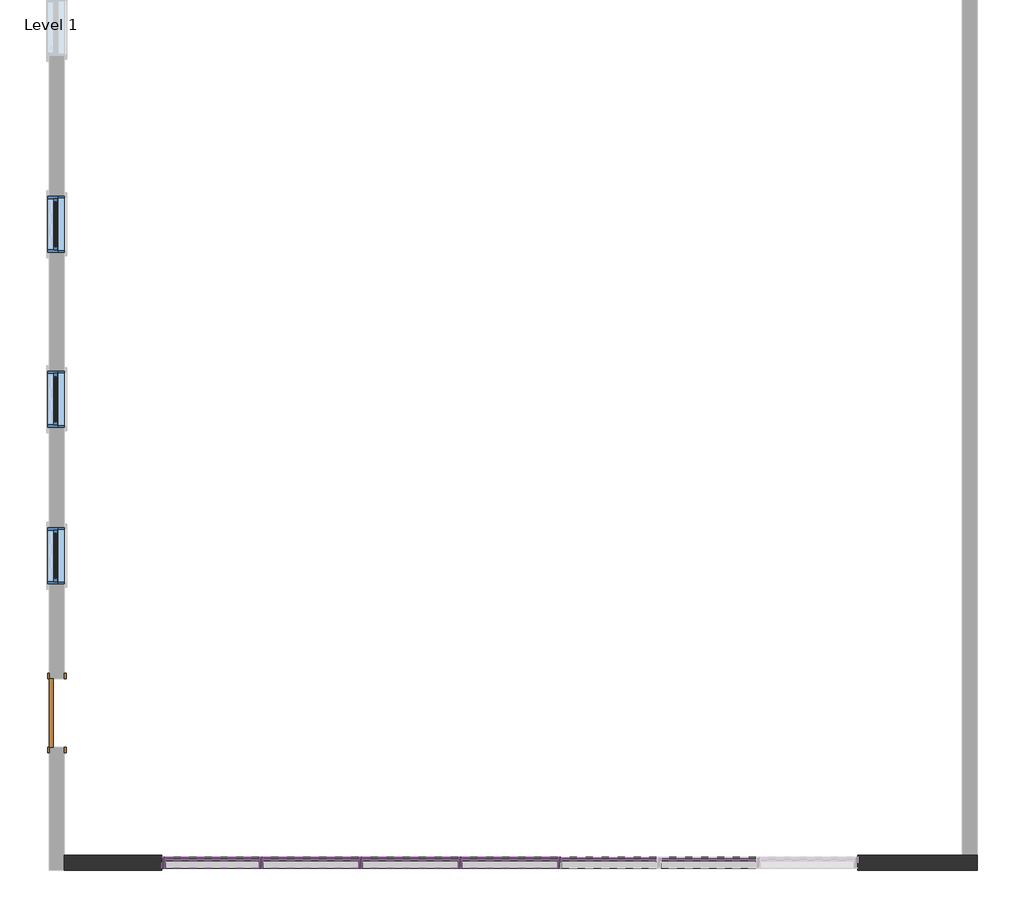
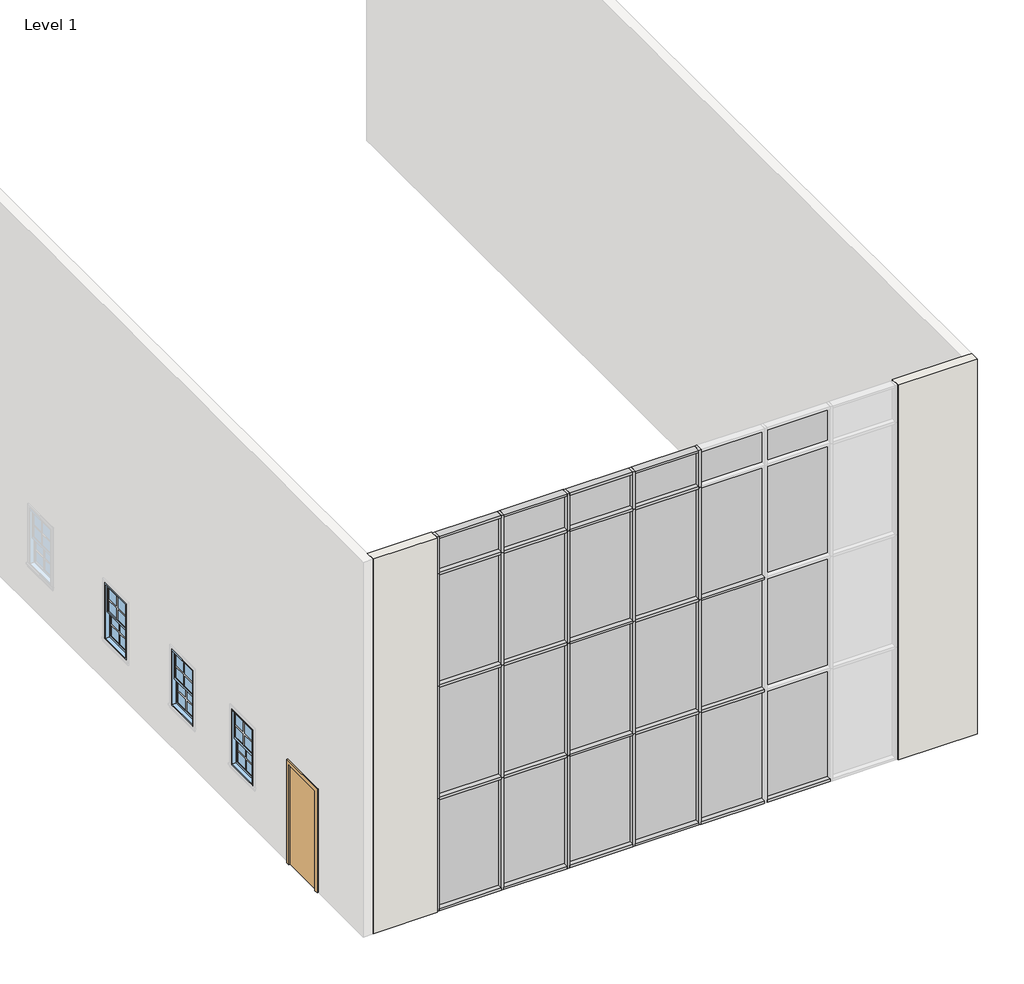
# One storey, part 1 of 2: 44 members, 24 plates, 3 windows, 1 door, 1 wall.
"""IFC4 building model written with IfcOpenShell, lengths in millimetres."""

import ifcopenshell
import ifcopenshell.guid

model = None  # the IFC model being written
_history = None  # IfcOwnerHistory: only IFC2X3 demands one
_inside = {}  # id of a spatial element -> (the spatial element, [elements in it])
_under = {}  # id of a project, library or spatial element -> (it, [spatial elements below it])
_declared = {}  # id of a project -> (the project, [libraries it declares])
_typed = {}  # id of a type object -> (the type object, [elements of that type])
_made_of = {}  # id of a material, layer set ... -> (it, [elements and type objects made of it])


def new_model(schema):
    """Start an empty IFC model of exactly this schema.

    Asked for "IFC4X3", IfcOpenShell would pick the latest addendum, in which some entities
    have other attributes; the version numbers below select the first issue.
    IFC2X3 requires an IfcOwnerHistory on every rooted entity: one is made here for all.
    """
    global model, _history
    if schema == "IFC4X3":
        model = ifcopenshell.file(schema_version=(4, 3, 0, 0))
    else:
        model = ifcopenshell.file(schema=schema)
    _inside.clear()
    _under.clear()
    _declared.clear()
    _typed.clear()
    _made_of.clear()
    _history = None
    if model.schema == "IFC2X3":
        org = make("IfcOrganization", Name="unknown")
        user = make(
            "IfcPersonAndOrganization",
            ThePerson=make("IfcPerson", FamilyName="unknown"),
            TheOrganization=org,
        )
        app = make(
            "IfcApplication",
            ApplicationDeveloper=org,
            Version="unknown",
            ApplicationFullName="unknown",
            ApplicationIdentifier="unknown",
        )
        _history = make(
            "IfcOwnerHistory",
            OwningUser=user,
            OwningApplication=app,
            ChangeAction="ADDED",
            CreationDate=0,
        )
    return model


def make(cls, **values):
    """One entity of the class cls with the attributes given. An attribute that is None is left unset."""
    return model.create_entity(
        cls, **{name: value for name, value in values.items() if value is not None}
    )


def rooted(cls, **values):
    """An entity with a GlobalId (a new one), such as an element, a storey or a relation."""
    return make(cls, GlobalId=ifcopenshell.guid.new(), OwnerHistory=_history, **values)


def si_unit(unit_type, name, prefix=None):
    """IfcSIUnit, for example si_unit("LENGTHUNIT", "METRE", prefix="MILLI")."""
    return make("IfcSIUnit", UnitType=unit_type, Prefix=prefix, Name=name)


def assignment(units):
    """IfcUnitAssignment: the units of a project."""
    return None if units is None else make("IfcUnitAssignment", Units=units)


def point(xyz):
    """IfcCartesianPoint."""
    return None if xyz is None else make("IfcCartesianPoint", Coordinates=xyz)


def direction(xyz):
    """IfcDirection."""
    return None if xyz is None else make("IfcDirection", DirectionRatios=xyz)


def frame(location, z_axis=None, x_axis=None):
    """IfcAxis2Placement3D, a coordinate frame: its origin and axes. An axis left out is left unset."""
    return make(
        "IfcAxis2Placement3D",
        Location=point(location),
        Axis=direction(z_axis),
        RefDirection=direction(x_axis),
    )


def origin():
    """The frame at (0, 0, 0) with its axes left unset."""
    return frame((0.0, 0.0, 0.0))


def origin_with_axes():
    """The frame at (0, 0, 0) with the z axis (0, 0, 1) and the x axis (1, 0, 0) written out."""
    return frame((0.0, 0.0, 0.0), z_axis=(0.0, 0.0, 1.0), x_axis=(1.0, 0.0, 0.0))


def place(relative_to, where):
    """IfcLocalPlacement: puts the frame where relative to a parent placement (None: the world)."""
    return make(
        "IfcLocalPlacement", PlacementRelTo=relative_to, RelativePlacement=where
    )


def context(
    kind, dimensions, precision=None, world=None, true_north=None, identifier=None
):
    """IfcGeometricRepresentationContext, for example the 3D "Model" context."""
    return make(
        "IfcGeometricRepresentationContext",
        ContextIdentifier=identifier,
        ContextType=kind,
        CoordinateSpaceDimension=dimensions,
        Precision=precision,
        WorldCoordinateSystem=world,
        TrueNorth=true_north,
    )


def project(units=None, contexts=None):
    """IfcProject with its units and contexts."""
    return rooted(
        "IfcProject",
        Name="project",
        RepresentationContexts=contexts,
        UnitsInContext=assignment(units),
    )


def spatial(cls, under=None, at=None, **own):
    """A site, building, storey or space (cls), placed at a placement, below another one or the project."""
    s = rooted(cls, ObjectPlacement=at, **own)
    if under is not None:
        _under.setdefault(under.id(), (under, []))[1].append(s)
    return s


def polyline(points):
    """IfcPolyline through the points."""
    return make("IfcPolyline", Points=[point(p) for p in points])


def outline(outer, holes=None, kind="AREA"):
    """IfcArbitraryClosedProfileDef: a profile drawn as a closed curve; with holes, ...WithVoids."""
    if holes is None:
        return make("IfcArbitraryClosedProfileDef", ProfileType=kind, OuterCurve=outer)
    return make(
        "IfcArbitraryProfileDefWithVoids",
        ProfileType=kind,
        OuterCurve=outer,
        InnerCurves=holes,
    )


def extrude(swept, where, along, depth):
    """IfcExtrudedAreaSolid: the profile swept, set in the frame where, extruded along a direction by depth."""
    return make(
        "IfcExtrudedAreaSolid",
        SweptArea=swept,
        Position=where,
        ExtrudedDirection=direction(along),
        Depth=depth,
    )


def faces_of(points, faces, orient=None, outer=None):
    """IfcFace entities. A face is a list of loops; a loop is a list of indices into points, from 0.

    orient and outer hold one flag for each loop. By default every Orientation is true, the
    first loop of a face is its IfcFaceOuterBound and the others are IfcFaceBound.
    """
    made = []
    for i, loops in enumerate(faces):
        bounds = []
        for j, loop in enumerate(loops):
            is_outer = j == 0 if outer is None else outer[i][j]
            bounds.append(
                make(
                    "IfcFaceOuterBound" if is_outer else "IfcFaceBound",
                    Bound=make("IfcPolyLoop", Polygon=[points[k] for k in loop]),
                    Orientation=True if orient is None else orient[i][j],
                )
            )
        made.append(make("IfcFace", Bounds=bounds))
    return made


def faceted_brep(points, faces, orient=None, outer=None, voids=None):
    """IfcFacetedBrep: a solid bounded by flat faces; with voids (closed shells), ...WithVoids."""
    shared = [point(p) for p in points]
    hull = make("IfcClosedShell", CfsFaces=faces_of(shared, faces, orient, outer))
    if voids is None:
        return make("IfcFacetedBrep", Outer=hull)
    return make(
        "IfcFacetedBrepWithVoids",
        Outer=hull,
        Voids=[
            make(cls, CfsFaces=faces_of(shared, fs, o, b)) for cls, fs, o, b in voids
        ],
    )


def shape(context_of_items, identifier, shape_type, items):
    """IfcShapeRepresentation: the items that make up one representation, for example the "Body"."""
    return make(
        "IfcShapeRepresentation",
        ContextOfItems=context_of_items,
        RepresentationIdentifier=identifier,
        RepresentationType=shape_type,
        Items=items,
    )


def source(mapping_origin, context_of_items, identifier, shape_type, items):
    """IfcRepresentationMap: a shape defined once, which mapped items show again and again."""
    return make(
        "IfcRepresentationMap",
        MappingOrigin=mapping_origin,
        MappedRepresentation=shape(context_of_items, identifier, shape_type, items),
    )


def transform(
    local_origin,
    x_axis=None,
    y_axis=None,
    z_axis=None,
    scale=None,
    scale2=None,
    scale3=None,
    uniform=True,
):
    """IfcCartesianTransformationOperator3D, or its non-uniform kind. x_axis, y_axis, z_axis: its Axis1, 2, 3."""
    if uniform:
        return make(
            "IfcCartesianTransformationOperator3D",
            Axis1=direction(x_axis),
            Axis2=direction(y_axis),
            LocalOrigin=point(local_origin),
            Scale=scale,
            Axis3=direction(z_axis),
        )
    return make(
        "IfcCartesianTransformationOperator3DnonUniform",
        Axis1=direction(x_axis),
        Axis2=direction(y_axis),
        LocalOrigin=point(local_origin),
        Scale=scale,
        Axis3=direction(z_axis),
        Scale2=scale2,
        Scale3=scale3,
    )


def mapped(mapping_source, mapping_target):
    """IfcMappedItem: shows the shape of a source again, moved by a transform."""
    return make(
        "IfcMappedItem", MappingSource=mapping_source, MappingTarget=mapping_target
    )


def made_of(thing, what):
    """Note that an element or type object is made of a material, layer set ...; save() writes the relation."""
    if what is not None:
        _made_of.setdefault(what.id(), (what, []))[1].append(thing)
    return thing


def element(
    cls,
    number,
    at=None,
    inside=None,
    cuts=None,
    type_object=None,
    material=None,
    context=None,
    identifier="Body",
    shape_type=None,
    held_by="IfcProductDefinitionShape",
    body=None,
    shapes=None,
    **own,
):
    """One element of the class cls, such as IfcWall. Its Tag is "e" and its number.

    at: its placement. inside: the storey or other place that contains it. cuts: it is an
    opening in that element (IfcRelVoidsElement). A single representation is given by context,
    identifier, shape_type and body (its items); several are given by shapes. held_by: the class
    of the entity that holds the representations. save() writes the other relations.
    """
    e = rooted(cls, Tag="e%d" % number, ObjectPlacement=at, **own)
    if body is not None:
        shapes = [shape(context, identifier, shape_type, body)]
    if shapes is not None:
        e.Representation = make(held_by, Representations=shapes)
    if inside is not None:
        _inside.setdefault(inside.id(), (inside, []))[1].append(e)
    if cuts is not None:
        rooted(
            "IfcRelVoidsElement", RelatingBuildingElement=cuts, RelatedOpeningElement=e
        )
    if type_object is not None:
        _typed.setdefault(type_object.id(), (type_object, []))[1].append(e)
    return made_of(e, material)


def aggregate(whole, parts):
    """IfcRelAggregates: a whole, such as a stair, and the parts it consists of."""
    return rooted("IfcRelAggregates", RelatingObject=whole, RelatedObjects=parts)


def save(model, path):
    """Write the relations noted so far, then the file.

    IfcRelAggregates (storeys below a building ...), IfcRelContainedInSpatialStructure (elements
    in a storey), IfcRelDefinesByType, IfcRelAssociatesMaterial and IfcRelDeclares: one each for
    every whole, place, type object, material and project.
    """
    for whole, parts in _under.values():
        aggregate(whole, parts)
    for where, things in _inside.values():
        rooted(
            "IfcRelContainedInSpatialStructure",
            RelatedElements=things,
            RelatingStructure=where,
        )
    for kind, things in _typed.values():
        rooted("IfcRelDefinesByType", RelatedObjects=things, RelatingType=kind)
    for what, things in _made_of.values():
        rooted("IfcRelAssociatesMaterial", RelatedObjects=things, RelatingMaterial=what)
    for by, libraries in _declared.values():
        rooted("IfcRelDeclares", RelatingContext=by, RelatedDefinitions=libraries)
    model.write(path)


def m_single_flush_0915_x_2134mm_6a9e8738(model_context):
    return source(origin(), model_context, "Body", "SweptSolid", [
        extrude(outline(polyline([(2210.0, -533.5), (0.0, -533.5), (0.0, -457.5), (2134.0, -457.5), (2134.0, 457.5), (0.0, 457.5), (0.0, 533.5), (2210.0, 533.5), (2210.0, -533.5)])), frame((0.0, 100.0, 0.0), z_axis=(0.0, 1.0, 0.0), x_axis=(0.0, 0.0, 1.0)), (0.0, 0.0, 1.0), 25.0),
        extrude(outline(polyline([(2210.0, 533.5), (2210.0, -533.5), (0.0, -533.5), (0.0, -457.5), (2134.0, -457.5), (2134.0, 457.5), (0.0, 457.5), (0.0, 533.5), (2210.0, 533.5)])), frame((0.0, -125.0, 0.0), z_axis=(0.0, 1.0, 0.0), x_axis=(0.0, 0.0, 1.0)), (0.0, 0.0, 1.0), 25.0),
        extrude(outline(polyline([(457.5, 49.0), (-457.5, 49.0), (-457.5, 100.0), (457.5, 100.0), (457.5, 49.0)])), origin_with_axes(), (0.0, 0.0, 1.0), 2134.0),
    ])


def rectangular_mullion_50mm_x_150mm_302a0cfa(model_context):
    return source(origin(), model_context, "Body", "SweptSolid", [
        extrude(outline(polyline([(0.0, 75.0), (0.0, -75.0), (-50.0, -75.0), (-50.0, 75.0), (0.0, 75.0)])), frame((0.0, 0.0, -1253.5714288), z_axis=(0.0, 0.0, 1.0), x_axis=(1.0, 0.0, 0.0)), (0.0, 0.0, 1.0), 1253.5714288),
    ])


def rectangular_mullion_50mm_x_150mm_11a5ee59(model_context):
    return source(origin(), model_context, "Body", "SweptSolid", [
        extrude(outline(polyline([(0.0, 75.0), (0.0, -75.0), (-50.0, -75.0), (-50.0, 75.0), (0.0, 75.0)])), frame((0.0, 0.0, -1278.5714285), z_axis=(0.0, 0.0, 1.0), x_axis=(1.0, 0.0, 0.0)), (0.0, 0.0, 1.0), 1278.5714285),
    ])


def rectangular_mullion_50mm_x_150mm_46426fc7(model_context):
    return source(origin(), model_context, "Body", "SweptSolid", [
        extrude(outline(polyline([(25.0, 75.0), (25.0, -75.0), (-25.0, -75.0), (-25.0, 75.0), (25.0, 75.0)])), frame((0.0, 0.0, -1253.5714288), z_axis=(0.0, 0.0, 1.0), x_axis=(1.0, 0.0, 0.0)), (0.0, 0.0, 1.0), 1253.5714288),
    ])


def rectangular_mullion_50mm_x_150mm_f38f42f6(model_context):
    return source(origin(), model_context, "Body", "SweptSolid", [
        extrude(outline(polyline([(25.0, 75.0), (25.0, -75.0), (-25.0, -75.0), (-25.0, 75.0), (25.0, 75.0)])), frame((0.0, 0.0, -1278.5714285), z_axis=(0.0, 0.0, 1.0), x_axis=(1.0, 0.0, 0.0)), (0.0, 0.0, 1.0), 1278.5714285),
    ])


def rectangular_mullion_50mm_x_150mm_6225e4e3(model_context):
    return source(origin(), model_context, "Body", "SweptSolid", [
        extrude(outline(polyline([(25.0, 75.0), (25.0, -75.0), (-25.0, -75.0), (-25.0, 75.0), (25.0, 75.0)])), frame((0.0, 0.0, -2400.0), z_axis=(0.0, 0.0, 1.0), x_axis=(1.0, 0.0, 0.0)), (0.0, 0.0, 1.0), 2400.0),
    ])


def rectangular_mullion_50mm_x_150mm_662c37b1(model_context):
    return source(origin(), model_context, "Body", "SweptSolid", [
        extrude(outline(polyline([(0.0, 75.0), (0.0, -75.0), (-50.0, -75.0), (-50.0, 75.0), (0.0, 75.0)])), frame((0.0, 0.0, -2400.0), z_axis=(0.0, 0.0, 1.0), x_axis=(1.0, 0.0, 0.0)), (0.0, 0.0, 1.0), 2400.0),
    ])


def rectangular_mullion_50mm_x_150mm_14f10ac7(model_context):
    return source(origin(), model_context, "Body", "SweptSolid", [
        extrude(outline(polyline([(25.0, 75.0), (25.0, -75.0), (-25.0, -75.0), (-25.0, 75.0), (25.0, 75.0)])), frame((0.0, 0.0, -800.0), z_axis=(0.0, 0.0, 1.0), x_axis=(1.0, 0.0, 0.0)), (0.0, 0.0, 1.0), 800.0),
    ])


def rectangular_mullion_50mm_x_150mm_6ffebc0f(model_context):
    return source(origin(), model_context, "Body", "SweptSolid", [
        extrude(outline(polyline([(0.0, 75.0), (0.0, -75.0), (-50.0, -75.0), (-50.0, 75.0), (0.0, 75.0)])), frame((0.0, 0.0, -800.0), z_axis=(0.0, 0.0, 1.0), x_axis=(1.0, 0.0, 0.0)), (0.0, 0.0, 1.0), 800.0),
    ])


def system_panel_glazed_b60b372a(model_context):
    return source(origin(), model_context, "Body", "SweptSolid", [
        extrude(outline(polyline([(626.7857144, 24.5), (-626.7857144, 24.5), (-626.7857144, 49.5), (626.7857144, 49.5), (626.7857144, 24.5)])), origin_with_axes(), (0.0, 0.0, 1.0), 2325.0),
    ])


def system_panel_glazed_fd68b2ce(model_context):
    return source(origin(), model_context, "Body", "SweptSolid", [
        extrude(outline(polyline([(639.2857142, 24.5), (-639.2857142, 24.5), (-639.2857142, 49.5), (639.2857142, 49.5), (639.2857142, 24.5)])), origin_with_axes(), (0.0, 0.0, 1.0), 2325.0),
    ])


def system_panel_glazed_eec4e8b3(model_context):
    return source(origin(), model_context, "Body", "SweptSolid", [
        extrude(outline(polyline([(626.7857144, 24.5), (-626.7857144, 24.5), (-626.7857144, 49.5), (626.7857144, 49.5), (626.7857144, 24.5)])), origin_with_axes(), (0.0, 0.0, 1.0), 2350.0),
    ])


def system_panel_glazed_5b896d3e(model_context):
    return source(origin(), model_context, "Body", "SweptSolid", [
        extrude(outline(polyline([(639.2857142, 24.5), (-639.2857142, 24.5), (-639.2857142, 49.5), (639.2857142, 49.5), (639.2857142, 24.5)])), origin_with_axes(), (0.0, 0.0, 1.0), 2350.0),
    ])


def system_panel_glazed_efd17426(model_context):
    return source(origin(), model_context, "Body", "SweptSolid", [
        extrude(outline(polyline([(626.7857144, 24.5), (-626.7857144, 24.5), (-626.7857144, 49.5), (626.7857144, 49.5), (626.7857144, 24.5)])), origin_with_axes(), (0.0, 0.0, 1.0), 725.0),
    ])


def system_panel_glazed_74448b90(model_context):
    return source(origin(), model_context, "Body", "SweptSolid", [
        extrude(outline(polyline([(639.2857142, 24.5), (-639.2857142, 24.5), (-639.2857142, 49.5), (639.2857142, 49.5), (639.2857142, 24.5)])), origin_with_axes(), (0.0, 0.0, 1.0), 725.0),
    ])


def m_window_double_hung_750_x_1200mm_41070976(model_context):
    return source(origin(), model_context, "Body", "SweptSolid", [
        extrude(outline(polyline([(298.8, 30.15), (298.8, 23.8), (-298.8, 23.8), (-298.8, 30.15), (298.8, 30.15)])), frame((0.0, 0.0, 990.6), z_axis=(0.0, 0.0, 1.0), x_axis=(1.0, 0.0, 0.0)), (0.0, 0.0, 1.0), 501.575),
        extrude(outline(polyline([(-298.8, 17.45), (298.8, 17.45), (298.8, 11.1), (-298.8, 11.1), (-298.8, 17.45)])), frame((0.0, 0.0, 990.6), z_axis=(0.0, 0.0, 1.0), x_axis=(1.0, 0.0, 0.0)), (0.0, 0.0, 1.0), 501.575),
        extrude(outline(polyline([(298.8, 74.6), (298.8, 68.25), (-298.8, 68.25), (-298.8, 74.6), (298.8, 74.6)])), frame((0.0, 0.0, 1536.625), z_axis=(0.0, 0.0, 1.0), x_axis=(1.0, 0.0, 0.0)), (0.0, 0.0, 1.0), 501.575),
        extrude(outline(polyline([(-298.8, 61.9), (298.8, 61.9), (298.8, 55.55), (-298.8, 55.55), (-298.8, 61.9)])), frame((0.0, 0.0, 1536.625), z_axis=(0.0, 0.0, 1.0), x_axis=(1.0, 0.0, 0.0)), (0.0, 0.0, 1.0), 501.575),
        extrude(outline(polyline([(1536.625, -343.25), (946.15, -343.25), (946.15, 343.25), (1536.625, 343.25), (1536.625, -343.25)]), holes=[polyline([(1492.175, 298.8), (990.6, 298.8), (990.6, -298.8), (1492.175, -298.8), (1492.175, 298.8)])]), frame((0.0, -1.6, 0.0), z_axis=(0.0, 1.0, 0.0), x_axis=(0.0, 0.0, 1.0)), (0.0, 0.0, 1.0), 44.45),
        extrude(outline(polyline([(2082.65, -343.25), (1492.175, -343.25), (1492.175, 343.25), (2082.65, 343.25), (2082.65, -343.25)]), holes=[polyline([(2038.2, 298.8), (1536.625, 298.8), (1536.625, -298.8), (2038.2, -298.8), (2038.2, 298.8)])]), frame((0.0, 42.85, 0.0), z_axis=(0.0, 1.0, 0.0), x_axis=(0.0, 0.0, 1.0)), (0.0, 0.0, 1.0), 44.45),
        extrude(outline(polyline([(2114.4, -375.0), (914.4, -375.0), (914.4, 375.0), (2114.4, 375.0), (2114.4, -375.0)]), holes=[polyline([(2082.65, 343.25), (946.15, 343.25), (946.15, -343.25), (2082.65, -343.25), (2082.65, 343.25)])]), frame((0.0, -14.3, 0.0), z_axis=(0.0, 1.0, 0.0), x_axis=(0.0, 0.0, 1.0)), (0.0, 0.0, 1.0), 133.35),
        extrude(outline(polyline([(2114.4, 375.0), (2114.4, -375.0), (914.4, -375.0), (914.4, 375.0), (2114.4, 375.0)]), holes=[polyline([(2095.35, 355.95), (933.45, 355.95), (933.45, -355.95), (2095.35, -355.95), (2095.35, 355.95)])]), frame((0.0, -100.0, 0.0), z_axis=(0.0, 1.0, 0.0), x_axis=(0.0, 0.0, 1.0)), (0.0, 0.0, 1.0), 85.7),
    ])


model = new_model("IFC4")

# Units and contexts
model_context = context("Model", 3, world=origin())
ifc_project = project(units=[si_unit("LENGTHUNIT", "METRE", prefix="MILLI")], contexts=[model_context])

# Site, building, storey
site = spatial("IfcSite", under=ifc_project)
building = spatial("IfcBuilding", under=site)
storey = spatial("IfcBuildingStorey", under=building, Name="Level 1", Elevation=0.0)

# Door
placement = place(None, origin())
m_single_flush_0915_x_2134mm_shape = m_single_flush_0915_x_2134mm_6a9e8738(model_context)
element("IfcDoor", 1, ObjectType="M_Single-Flush : 0915 x 2134mm", at=placement, inside=storey, context=model_context, shape_type="MappedRepresentation", body=[
    mapped(m_single_flush_0915_x_2134mm_shape, transform((-6967.834392, -6666.9793434, 0.0), x_axis=(0.0, 1.0, 0.0), y_axis=(-1.0, 0.0, 0.0), z_axis=(0.0, 0.0, 1.0))),
])

# Members
rectangular_mullion_50mm_x_150mm_shape = rectangular_mullion_50mm_x_150mm_302a0cfa(model_context)
element("IfcMember", 2, ObjectType="Rectangular Mullion : 50mm x 150mm", at=placement, inside=storey, context=model_context, shape_type="MappedRepresentation", body=[
    mapped(rectangular_mullion_50mm_x_150mm_shape, transform((-5517.834392, -8666.9793434, 0.0), x_axis=(0.0, 0.0, -1.0), y_axis=(0.0, -1.0, 0.0), z_axis=(-1.0, 0.0, 0.0))),
])
rectangular_mullion_50mm_x_150mm_2_shape = rectangular_mullion_50mm_x_150mm_11a5ee59(model_context)
element("IfcMember", 3, ObjectType="Rectangular Mullion : 50mm x 150mm", at=placement, inside=storey, context=model_context, shape_type="MappedRepresentation", body=[
    mapped(rectangular_mullion_50mm_x_150mm_2_shape, transform((-4214.2629632, -8666.9793434, 0.0), x_axis=(0.0, 0.0, -1.0), y_axis=(0.0, -1.0, 0.0), z_axis=(-1.0, 0.0, 0.0))),
])
element("IfcMember", 4, ObjectType="Rectangular Mullion : 50mm x 150mm", at=placement, inside=storey, context=model_context, shape_type="MappedRepresentation", body=[
    mapped(rectangular_mullion_50mm_x_150mm_2_shape, transform((-2885.6915347, -8666.9793434, 0.0), x_axis=(0.0, 0.0, -1.0), y_axis=(0.0, -1.0, 0.0), z_axis=(-1.0, 0.0, 0.0))),
])
element("IfcMember", 5, ObjectType="Rectangular Mullion : 50mm x 150mm", at=placement, inside=storey, context=model_context, shape_type="MappedRepresentation", body=[
    mapped(rectangular_mullion_50mm_x_150mm_2_shape, transform((-1557.1201062, -8666.9793434, 0.0), x_axis=(0.0, 0.0, -1.0), y_axis=(0.0, -1.0, 0.0), z_axis=(-1.0, 0.0, 0.0))),
])
element("IfcMember", 6, ObjectType="Rectangular Mullion : 50mm x 150mm", at=placement, inside=storey, context=model_context, shape_type="MappedRepresentation", body=[
    mapped(rectangular_mullion_50mm_x_150mm_2_shape, transform((-228.5486777, -8666.9793434, 0.0), x_axis=(0.0, 0.0, -1.0), y_axis=(0.0, -1.0, 0.0), z_axis=(-1.0, 0.0, 0.0))),
])
element("IfcMember", 7, ObjectType="Rectangular Mullion : 50mm x 150mm", at=placement, inside=storey, context=model_context, shape_type="MappedRepresentation", body=[
    mapped(rectangular_mullion_50mm_x_150mm_2_shape, transform((1100.0227508, -8666.9793434, 0.0), x_axis=(0.0, 0.0, -1.0), y_axis=(0.0, -1.0, 0.0), z_axis=(-1.0, 0.0, 0.0))),
])
rectangular_mullion_50mm_x_150mm_3_shape = rectangular_mullion_50mm_x_150mm_46426fc7(model_context)
element("IfcMember", 8, ObjectType="Rectangular Mullion : 50mm x 150mm", at=placement, inside=storey, context=model_context, shape_type="MappedRepresentation", body=[
    mapped(rectangular_mullion_50mm_x_150mm_3_shape, transform((-4264.2629632, -8666.9793434, 2400.0), x_axis=(0.0, 0.0, 1.0), y_axis=(0.0, -1.0, 0.0), z_axis=(1.0, 0.0, 0.0))),
])
element("IfcMember", 9, ObjectType="Rectangular Mullion : 50mm x 150mm", at=placement, inside=storey, context=model_context, shape_type="MappedRepresentation", body=[
    mapped(rectangular_mullion_50mm_x_150mm_3_shape, transform((-4264.2629632, -8666.9793434, 4800.0), x_axis=(0.0, 0.0, 1.0), y_axis=(0.0, -1.0, 0.0), z_axis=(1.0, 0.0, 0.0))),
])
element("IfcMember", 10, ObjectType="Rectangular Mullion : 50mm x 150mm", at=placement, inside=storey, context=model_context, shape_type="MappedRepresentation", body=[
    mapped(rectangular_mullion_50mm_x_150mm_3_shape, transform((-4264.2629632, -8666.9793434, 7200.0), x_axis=(0.0, 0.0, 1.0), y_axis=(0.0, -1.0, 0.0), z_axis=(1.0, 0.0, 0.0))),
])
rectangular_mullion_50mm_x_150mm_4_shape = rectangular_mullion_50mm_x_150mm_f38f42f6(model_context)
element("IfcMember", 11, ObjectType="Rectangular Mullion : 50mm x 150mm", at=placement, inside=storey, context=model_context, shape_type="MappedRepresentation", body=[
    mapped(rectangular_mullion_50mm_x_150mm_4_shape, transform((-2935.6915347, -8666.9793434, 2400.0), x_axis=(0.0, 0.0, 1.0), y_axis=(0.0, -1.0, 0.0), z_axis=(1.0, 0.0, 0.0))),
])
element("IfcMember", 12, ObjectType="Rectangular Mullion : 50mm x 150mm", at=placement, inside=storey, context=model_context, shape_type="MappedRepresentation", body=[
    mapped(rectangular_mullion_50mm_x_150mm_4_shape, transform((-1607.1201062, -8666.9793434, 2400.0), x_axis=(0.0, 0.0, 1.0), y_axis=(0.0, -1.0, 0.0), z_axis=(1.0, 0.0, 0.0))),
])
element("IfcMember", 13, ObjectType="Rectangular Mullion : 50mm x 150mm", at=placement, inside=storey, context=model_context, shape_type="MappedRepresentation", body=[
    mapped(rectangular_mullion_50mm_x_150mm_4_shape, transform((-278.5486777, -8666.9793434, 2400.0), x_axis=(0.0, 0.0, 1.0), y_axis=(0.0, -1.0, 0.0), z_axis=(1.0, 0.0, 0.0))),
])
element("IfcMember", 14, ObjectType="Rectangular Mullion : 50mm x 150mm", at=placement, inside=storey, context=model_context, shape_type="MappedRepresentation", body=[
    mapped(rectangular_mullion_50mm_x_150mm_4_shape, transform((1050.0227508, -8666.9793434, 2400.0), x_axis=(0.0, 0.0, 1.0), y_axis=(0.0, -1.0, 0.0), z_axis=(1.0, 0.0, 0.0))),
])
element("IfcMember", 15, ObjectType="Rectangular Mullion : 50mm x 150mm", at=placement, inside=storey, context=model_context, shape_type="MappedRepresentation", body=[
    mapped(rectangular_mullion_50mm_x_150mm_4_shape, transform((-2935.6915347, -8666.9793434, 4800.0), x_axis=(0.0, 0.0, 1.0), y_axis=(0.0, -1.0, 0.0), z_axis=(1.0, 0.0, 0.0))),
])
element("IfcMember", 16, ObjectType="Rectangular Mullion : 50mm x 150mm", at=placement, inside=storey, context=model_context, shape_type="MappedRepresentation", body=[
    mapped(rectangular_mullion_50mm_x_150mm_4_shape, transform((-1607.1201062, -8666.9793434, 4800.0), x_axis=(0.0, 0.0, 1.0), y_axis=(0.0, -1.0, 0.0), z_axis=(1.0, 0.0, 0.0))),
])
element("IfcMember", 17, ObjectType="Rectangular Mullion : 50mm x 150mm", at=placement, inside=storey, context=model_context, shape_type="MappedRepresentation", body=[
    mapped(rectangular_mullion_50mm_x_150mm_4_shape, transform((-278.5486777, -8666.9793434, 4800.0), x_axis=(0.0, 0.0, 1.0), y_axis=(0.0, -1.0, 0.0), z_axis=(1.0, 0.0, 0.0))),
])
element("IfcMember", 18, ObjectType="Rectangular Mullion : 50mm x 150mm", at=placement, inside=storey, context=model_context, shape_type="MappedRepresentation", body=[
    mapped(rectangular_mullion_50mm_x_150mm_4_shape, transform((1050.0227508, -8666.9793434, 4800.0), x_axis=(0.0, 0.0, 1.0), y_axis=(0.0, -1.0, 0.0), z_axis=(1.0, 0.0, 0.0))),
])
element("IfcMember", 19, ObjectType="Rectangular Mullion : 50mm x 150mm", at=placement, inside=storey, context=model_context, shape_type="MappedRepresentation", body=[
    mapped(rectangular_mullion_50mm_x_150mm_4_shape, transform((-1607.1201062, -8666.9793434, 7200.0), x_axis=(0.0, 0.0, 1.0), y_axis=(0.0, -1.0, 0.0), z_axis=(1.0, 0.0, 0.0))),
])
element("IfcMember", 20, ObjectType="Rectangular Mullion : 50mm x 150mm", at=placement, inside=storey, context=model_context, shape_type="MappedRepresentation", body=[
    mapped(rectangular_mullion_50mm_x_150mm_4_shape, transform((-278.5486777, -8666.9793434, 7200.0), x_axis=(0.0, 0.0, 1.0), y_axis=(0.0, -1.0, 0.0), z_axis=(1.0, 0.0, 0.0))),
])
element("IfcMember", 21, ObjectType="Rectangular Mullion : 50mm x 150mm", at=placement, inside=storey, context=model_context, shape_type="MappedRepresentation", body=[
    mapped(rectangular_mullion_50mm_x_150mm_4_shape, transform((-2935.6915347, -8666.9793434, 7200.0), x_axis=(0.0, 0.0, 1.0), y_axis=(0.0, -1.0, 0.0), z_axis=(1.0, 0.0, 0.0))),
])
rectangular_mullion_50mm_x_150mm_5_shape = rectangular_mullion_50mm_x_150mm_6225e4e3(model_context)
element("IfcMember", 22, ObjectType="Rectangular Mullion : 50mm x 150mm", at=placement, inside=storey, context=model_context, shape_type="MappedRepresentation", body=[
    mapped(rectangular_mullion_50mm_x_150mm_5_shape, transform((-4239.2629632, -8666.9793434, 0.0), x_axis=(1.0, 0.0, 0.0), y_axis=(0.0, -1.0, 0.0), z_axis=(0.0, 0.0, -1.0))),
])
element("IfcMember", 23, ObjectType="Rectangular Mullion : 50mm x 150mm", at=placement, inside=storey, context=model_context, shape_type="MappedRepresentation", body=[
    mapped(rectangular_mullion_50mm_x_150mm_5_shape, transform((-2910.6915347, -8666.9793434, 0.0), x_axis=(1.0, 0.0, 0.0), y_axis=(0.0, -1.0, 0.0), z_axis=(0.0, 0.0, -1.0))),
])
element("IfcMember", 24, ObjectType="Rectangular Mullion : 50mm x 150mm", at=placement, inside=storey, context=model_context, shape_type="MappedRepresentation", body=[
    mapped(rectangular_mullion_50mm_x_150mm_5_shape, transform((-1582.1201062, -8666.9793434, 0.0), x_axis=(1.0, 0.0, 0.0), y_axis=(0.0, -1.0, 0.0), z_axis=(0.0, 0.0, -1.0))),
])
element("IfcMember", 25, ObjectType="Rectangular Mullion : 50mm x 150mm", at=placement, inside=storey, context=model_context, shape_type="MappedRepresentation", body=[
    mapped(rectangular_mullion_50mm_x_150mm_5_shape, transform((-253.5486777, -8666.9793434, 0.0), x_axis=(1.0, 0.0, 0.0), y_axis=(0.0, -1.0, 0.0), z_axis=(0.0, 0.0, -1.0))),
])
element("IfcMember", 26, ObjectType="Rectangular Mullion : 50mm x 150mm", at=placement, inside=storey, context=model_context, shape_type="MappedRepresentation", body=[
    mapped(rectangular_mullion_50mm_x_150mm_5_shape, transform((-4239.2629632, -8666.9793434, 2400.0), x_axis=(1.0, 0.0, 0.0), y_axis=(0.0, -1.0, 0.0), z_axis=(0.0, 0.0, -1.0))),
])
element("IfcMember", 27, ObjectType="Rectangular Mullion : 50mm x 150mm", at=placement, inside=storey, context=model_context, shape_type="MappedRepresentation", body=[
    mapped(rectangular_mullion_50mm_x_150mm_5_shape, transform((-2910.6915347, -8666.9793434, 2400.0), x_axis=(1.0, 0.0, 0.0), y_axis=(0.0, -1.0, 0.0), z_axis=(0.0, 0.0, -1.0))),
])
element("IfcMember", 28, ObjectType="Rectangular Mullion : 50mm x 150mm", at=placement, inside=storey, context=model_context, shape_type="MappedRepresentation", body=[
    mapped(rectangular_mullion_50mm_x_150mm_5_shape, transform((-1582.1201062, -8666.9793434, 2400.0), x_axis=(1.0, 0.0, 0.0), y_axis=(0.0, -1.0, 0.0), z_axis=(0.0, 0.0, -1.0))),
])
element("IfcMember", 29, ObjectType="Rectangular Mullion : 50mm x 150mm", at=placement, inside=storey, context=model_context, shape_type="MappedRepresentation", body=[
    mapped(rectangular_mullion_50mm_x_150mm_5_shape, transform((-253.5486777, -8666.9793434, 2400.0), x_axis=(1.0, 0.0, 0.0), y_axis=(0.0, -1.0, 0.0), z_axis=(0.0, 0.0, -1.0))),
])
element("IfcMember", 30, ObjectType="Rectangular Mullion : 50mm x 150mm", at=placement, inside=storey, context=model_context, shape_type="MappedRepresentation", body=[
    mapped(rectangular_mullion_50mm_x_150mm_5_shape, transform((-4239.2629632, -8666.9793434, 4800.0), x_axis=(1.0, 0.0, 0.0), y_axis=(0.0, -1.0, 0.0), z_axis=(0.0, 0.0, -1.0))),
])
element("IfcMember", 31, ObjectType="Rectangular Mullion : 50mm x 150mm", at=placement, inside=storey, context=model_context, shape_type="MappedRepresentation", body=[
    mapped(rectangular_mullion_50mm_x_150mm_5_shape, transform((-2910.6915347, -8666.9793434, 4800.0), x_axis=(1.0, 0.0, 0.0), y_axis=(0.0, -1.0, 0.0), z_axis=(0.0, 0.0, -1.0))),
])
element("IfcMember", 32, ObjectType="Rectangular Mullion : 50mm x 150mm", at=placement, inside=storey, context=model_context, shape_type="MappedRepresentation", body=[
    mapped(rectangular_mullion_50mm_x_150mm_5_shape, transform((-1582.1201062, -8666.9793434, 4800.0), x_axis=(1.0, 0.0, 0.0), y_axis=(0.0, -1.0, 0.0), z_axis=(0.0, 0.0, -1.0))),
])
element("IfcMember", 33, ObjectType="Rectangular Mullion : 50mm x 150mm", at=placement, inside=storey, context=model_context, shape_type="MappedRepresentation", body=[
    mapped(rectangular_mullion_50mm_x_150mm_5_shape, transform((-253.5486777, -8666.9793434, 4800.0), x_axis=(1.0, 0.0, 0.0), y_axis=(0.0, -1.0, 0.0), z_axis=(0.0, 0.0, -1.0))),
])
rectangular_mullion_50mm_x_150mm_6_shape = rectangular_mullion_50mm_x_150mm_662c37b1(model_context)
element("IfcMember", 34, ObjectType="Rectangular Mullion : 50mm x 150mm", at=placement, inside=storey, context=model_context, shape_type="MappedRepresentation", body=[
    mapped(rectangular_mullion_50mm_x_150mm_6_shape, transform((-5567.834392, -8666.9793434, 2400.0), x_axis=(-1.0, 0.0, 0.0), y_axis=(0.0, -1.0, 0.0), z_axis=(0.0, 0.0, 1.0))),
])
element("IfcMember", 35, ObjectType="Rectangular Mullion : 50mm x 150mm", at=placement, inside=storey, context=model_context, shape_type="MappedRepresentation", body=[
    mapped(rectangular_mullion_50mm_x_150mm_6_shape, transform((-5567.834392, -8666.9793434, 4800.0), x_axis=(-1.0, 0.0, 0.0), y_axis=(0.0, -1.0, 0.0), z_axis=(0.0, 0.0, 1.0))),
])
element("IfcMember", 36, ObjectType="Rectangular Mullion : 50mm x 150mm", at=placement, inside=storey, context=model_context, shape_type="MappedRepresentation", body=[
    mapped(rectangular_mullion_50mm_x_150mm_6_shape, transform((-5567.834392, -8666.9793434, 7200.0), x_axis=(-1.0, 0.0, 0.0), y_axis=(0.0, -1.0, 0.0), z_axis=(0.0, 0.0, 1.0))),
])
rectangular_mullion_50mm_x_150mm_7_shape = rectangular_mullion_50mm_x_150mm_14f10ac7(model_context)
element("IfcMember", 37, ObjectType="Rectangular Mullion : 50mm x 150mm", at=placement, inside=storey, context=model_context, shape_type="MappedRepresentation", body=[
    mapped(rectangular_mullion_50mm_x_150mm_7_shape, transform((-1582.1201062, -8666.9793434, 7200.0), x_axis=(1.0, 0.0, 0.0), y_axis=(0.0, -1.0, 0.0), z_axis=(0.0, 0.0, -1.0))),
])
element("IfcMember", 38, ObjectType="Rectangular Mullion : 50mm x 150mm", at=placement, inside=storey, context=model_context, shape_type="MappedRepresentation", body=[
    mapped(rectangular_mullion_50mm_x_150mm_7_shape, transform((-253.5486777, -8666.9793434, 7200.0), x_axis=(1.0, 0.0, 0.0), y_axis=(0.0, -1.0, 0.0), z_axis=(0.0, 0.0, -1.0))),
])
element("IfcMember", 39, ObjectType="Rectangular Mullion : 50mm x 150mm", at=placement, inside=storey, context=model_context, shape_type="MappedRepresentation", body=[
    mapped(rectangular_mullion_50mm_x_150mm_7_shape, transform((-4239.2629632, -8666.9793434, 7200.0), x_axis=(1.0, 0.0, 0.0), y_axis=(0.0, -1.0, 0.0), z_axis=(0.0, 0.0, -1.0))),
])
element("IfcMember", 40, ObjectType="Rectangular Mullion : 50mm x 150mm", at=placement, inside=storey, context=model_context, shape_type="MappedRepresentation", body=[
    mapped(rectangular_mullion_50mm_x_150mm_7_shape, transform((-2910.6915347, -8666.9793434, 7200.0), x_axis=(1.0, 0.0, 0.0), y_axis=(0.0, -1.0, 0.0), z_axis=(0.0, 0.0, -1.0))),
])
element("IfcMember", 41, ObjectType="Rectangular Mullion : 50mm x 150mm", at=placement, inside=storey, context=model_context, shape_type="MappedRepresentation", body=[
    mapped(rectangular_mullion_50mm_x_150mm_shape, transform((-4264.2629632, -8666.9793434, 8000.0), x_axis=(0.0, 0.0, 1.0), y_axis=(0.0, -1.0, 0.0), z_axis=(1.0, 0.0, 0.0))),
])
element("IfcMember", 42, ObjectType="Rectangular Mullion : 50mm x 150mm", at=placement, inside=storey, context=model_context, shape_type="MappedRepresentation", body=[
    mapped(rectangular_mullion_50mm_x_150mm_2_shape, transform((-2935.6915347, -8666.9793434, 8000.0), x_axis=(0.0, 0.0, 1.0), y_axis=(0.0, -1.0, 0.0), z_axis=(1.0, 0.0, 0.0))),
])
element("IfcMember", 43, ObjectType="Rectangular Mullion : 50mm x 150mm", at=placement, inside=storey, context=model_context, shape_type="MappedRepresentation", body=[
    mapped(rectangular_mullion_50mm_x_150mm_2_shape, transform((-1607.1201062, -8666.9793434, 8000.0), x_axis=(0.0, 0.0, 1.0), y_axis=(0.0, -1.0, 0.0), z_axis=(1.0, 0.0, 0.0))),
])
element("IfcMember", 44, ObjectType="Rectangular Mullion : 50mm x 150mm", at=placement, inside=storey, context=model_context, shape_type="MappedRepresentation", body=[
    mapped(rectangular_mullion_50mm_x_150mm_2_shape, transform((-278.5486777, -8666.9793434, 8000.0), x_axis=(0.0, 0.0, 1.0), y_axis=(0.0, -1.0, 0.0), z_axis=(1.0, 0.0, 0.0))),
])
rectangular_mullion_50mm_x_150mm_8_shape = rectangular_mullion_50mm_x_150mm_6ffebc0f(model_context)
element("IfcMember", 45, ObjectType="Rectangular Mullion : 50mm x 150mm", at=placement, inside=storey, context=model_context, shape_type="MappedRepresentation", body=[
    mapped(rectangular_mullion_50mm_x_150mm_8_shape, transform((-5567.834392, -8666.9793434, 8000.0), x_axis=(-1.0, 0.0, 0.0), y_axis=(0.0, -1.0, 0.0), z_axis=(0.0, 0.0, 1.0))),
])

# Plates
system_panel_glazed_shape = system_panel_glazed_b60b372a(model_context)
element("IfcPlate", 46, ObjectType="System Panel : Glazed", at=placement, inside=storey, context=model_context, shape_type="MappedRepresentation", body=[
    mapped(system_panel_glazed_shape, transform((-4891.0486776, -8666.9793434, 50.0), x_axis=(1.0, 0.0, 0.0), y_axis=(0.0, 1.0, 0.0), z_axis=(0.0, 0.0, 1.0))),
])
system_panel_glazed_2_shape = system_panel_glazed_fd68b2ce(model_context)
element("IfcPlate", 47, ObjectType="System Panel : Glazed", at=placement, inside=storey, context=model_context, shape_type="MappedRepresentation", body=[
    mapped(system_panel_glazed_2_shape, transform((-3574.9772489, -8666.9793434, 50.0), x_axis=(1.0, 0.0, 0.0), y_axis=(0.0, 1.0, 0.0), z_axis=(0.0, 0.0, 1.0))),
])
element("IfcPlate", 48, ObjectType="System Panel : Glazed", at=placement, inside=storey, context=model_context, shape_type="MappedRepresentation", body=[
    mapped(system_panel_glazed_2_shape, transform((-2246.4058204, -8666.9793434, 50.0), x_axis=(1.0, 0.0, 0.0), y_axis=(0.0, 1.0, 0.0), z_axis=(0.0, 0.0, 1.0))),
])
element("IfcPlate", 49, ObjectType="System Panel : Glazed", at=placement, inside=storey, context=model_context, shape_type="MappedRepresentation", body=[
    mapped(system_panel_glazed_2_shape, transform((-917.834392, -8666.9793434, 50.0), x_axis=(1.0, 0.0, 0.0), y_axis=(0.0, 1.0, 0.0), z_axis=(0.0, 0.0, 1.0))),
])
element("IfcPlate", 50, ObjectType="System Panel : Glazed", at=placement, inside=storey, context=model_context, shape_type="MappedRepresentation", body=[
    mapped(system_panel_glazed_2_shape, transform((410.7370365, -8666.9793434, 50.0), x_axis=(1.0, 0.0, 0.0), y_axis=(0.0, 1.0, 0.0), z_axis=(0.0, 0.0, 1.0))),
])
element("IfcPlate", 51, ObjectType="System Panel : Glazed", at=placement, inside=storey, context=model_context, shape_type="MappedRepresentation", body=[
    mapped(system_panel_glazed_2_shape, transform((1739.308465, -8666.9793434, 50.0), x_axis=(1.0, 0.0, 0.0), y_axis=(0.0, 1.0, 0.0), z_axis=(0.0, 0.0, 1.0))),
])
system_panel_glazed_3_shape = system_panel_glazed_eec4e8b3(model_context)
element("IfcPlate", 52, ObjectType="System Panel : Glazed", at=placement, inside=storey, context=model_context, shape_type="MappedRepresentation", body=[
    mapped(system_panel_glazed_3_shape, transform((-4891.0486776, -8666.9793434, 2425.0), x_axis=(1.0, 0.0, 0.0), y_axis=(0.0, 1.0, 0.0), z_axis=(0.0, 0.0, 1.0))),
])
element("IfcPlate", 53, ObjectType="System Panel : Glazed", at=placement, inside=storey, context=model_context, shape_type="MappedRepresentation", body=[
    mapped(system_panel_glazed_3_shape, transform((-4891.0486776, -8666.9793434, 4825.0), x_axis=(1.0, 0.0, 0.0), y_axis=(0.0, 1.0, 0.0), z_axis=(0.0, 0.0, 1.0))),
])
system_panel_glazed_4_shape = system_panel_glazed_5b896d3e(model_context)
element("IfcPlate", 54, ObjectType="System Panel : Glazed", at=placement, inside=storey, context=model_context, shape_type="MappedRepresentation", body=[
    mapped(system_panel_glazed_4_shape, transform((-3574.9772489, -8666.9793434, 2425.0), x_axis=(1.0, 0.0, 0.0), y_axis=(0.0, 1.0, 0.0), z_axis=(0.0, 0.0, 1.0))),
])
element("IfcPlate", 55, ObjectType="System Panel : Glazed", at=placement, inside=storey, context=model_context, shape_type="MappedRepresentation", body=[
    mapped(system_panel_glazed_4_shape, transform((-2246.4058204, -8666.9793434, 2425.0), x_axis=(1.0, 0.0, 0.0), y_axis=(0.0, 1.0, 0.0), z_axis=(0.0, 0.0, 1.0))),
])
element("IfcPlate", 56, ObjectType="System Panel : Glazed", at=placement, inside=storey, context=model_context, shape_type="MappedRepresentation", body=[
    mapped(system_panel_glazed_4_shape, transform((-917.834392, -8666.9793434, 2425.0), x_axis=(1.0, 0.0, 0.0), y_axis=(0.0, 1.0, 0.0), z_axis=(0.0, 0.0, 1.0))),
])
element("IfcPlate", 57, ObjectType="System Panel : Glazed", at=placement, inside=storey, context=model_context, shape_type="MappedRepresentation", body=[
    mapped(system_panel_glazed_4_shape, transform((410.7370365, -8666.9793434, 2425.0), x_axis=(1.0, 0.0, 0.0), y_axis=(0.0, 1.0, 0.0), z_axis=(0.0, 0.0, 1.0))),
])
element("IfcPlate", 58, ObjectType="System Panel : Glazed", at=placement, inside=storey, context=model_context, shape_type="MappedRepresentation", body=[
    mapped(system_panel_glazed_4_shape, transform((1739.308465, -8666.9793434, 2425.0), x_axis=(1.0, 0.0, 0.0), y_axis=(0.0, 1.0, 0.0), z_axis=(0.0, 0.0, 1.0))),
])
element("IfcPlate", 59, ObjectType="System Panel : Glazed", at=placement, inside=storey, context=model_context, shape_type="MappedRepresentation", body=[
    mapped(system_panel_glazed_4_shape, transform((-3574.9772489, -8666.9793434, 4825.0), x_axis=(1.0, 0.0, 0.0), y_axis=(0.0, 1.0, 0.0), z_axis=(0.0, 0.0, 1.0))),
])
element("IfcPlate", 60, ObjectType="System Panel : Glazed", at=placement, inside=storey, context=model_context, shape_type="MappedRepresentation", body=[
    mapped(system_panel_glazed_4_shape, transform((-2246.4058204, -8666.9793434, 4825.0), x_axis=(1.0, 0.0, 0.0), y_axis=(0.0, 1.0, 0.0), z_axis=(0.0, 0.0, 1.0))),
])
element("IfcPlate", 61, ObjectType="System Panel : Glazed", at=placement, inside=storey, context=model_context, shape_type="MappedRepresentation", body=[
    mapped(system_panel_glazed_4_shape, transform((-917.834392, -8666.9793434, 4825.0), x_axis=(1.0, 0.0, 0.0), y_axis=(0.0, 1.0, 0.0), z_axis=(0.0, 0.0, 1.0))),
])
element("IfcPlate", 62, ObjectType="System Panel : Glazed", at=placement, inside=storey, context=model_context, shape_type="MappedRepresentation", body=[
    mapped(system_panel_glazed_4_shape, transform((410.7370365, -8666.9793434, 4825.0), x_axis=(1.0, 0.0, 0.0), y_axis=(0.0, 1.0, 0.0), z_axis=(0.0, 0.0, 1.0))),
])
element("IfcPlate", 63, ObjectType="System Panel : Glazed", at=placement, inside=storey, context=model_context, shape_type="MappedRepresentation", body=[
    mapped(system_panel_glazed_4_shape, transform((1739.308465, -8666.9793434, 4825.0), x_axis=(1.0, 0.0, 0.0), y_axis=(0.0, 1.0, 0.0), z_axis=(0.0, 0.0, 1.0))),
])
system_panel_glazed_5_shape = system_panel_glazed_efd17426(model_context)
element("IfcPlate", 64, ObjectType="System Panel : Glazed", at=placement, inside=storey, context=model_context, shape_type="MappedRepresentation", body=[
    mapped(system_panel_glazed_5_shape, transform((-4891.0486776, -8666.9793434, 7225.0), x_axis=(1.0, 0.0, 0.0), y_axis=(0.0, 1.0, 0.0), z_axis=(0.0, 0.0, 1.0))),
])
system_panel_glazed_6_shape = system_panel_glazed_74448b90(model_context)
element("IfcPlate", 65, ObjectType="System Panel : Glazed", at=placement, inside=storey, context=model_context, shape_type="MappedRepresentation", body=[
    mapped(system_panel_glazed_6_shape, transform((-3574.9772489, -8666.9793434, 7225.0), x_axis=(1.0, 0.0, 0.0), y_axis=(0.0, 1.0, 0.0), z_axis=(0.0, 0.0, 1.0))),
])
element("IfcPlate", 66, ObjectType="System Panel : Glazed", at=placement, inside=storey, context=model_context, shape_type="MappedRepresentation", body=[
    mapped(system_panel_glazed_6_shape, transform((-2246.4058204, -8666.9793434, 7225.0), x_axis=(1.0, 0.0, 0.0), y_axis=(0.0, 1.0, 0.0), z_axis=(0.0, 0.0, 1.0))),
])
element("IfcPlate", 67, ObjectType="System Panel : Glazed", at=placement, inside=storey, context=model_context, shape_type="MappedRepresentation", body=[
    mapped(system_panel_glazed_6_shape, transform((-917.834392, -8666.9793434, 7225.0), x_axis=(1.0, 0.0, 0.0), y_axis=(0.0, 1.0, 0.0), z_axis=(0.0, 0.0, 1.0))),
])
element("IfcPlate", 68, ObjectType="System Panel : Glazed", at=placement, inside=storey, context=model_context, shape_type="MappedRepresentation", body=[
    mapped(system_panel_glazed_6_shape, transform((410.7370365, -8666.9793434, 7225.0), x_axis=(1.0, 0.0, 0.0), y_axis=(0.0, 1.0, 0.0), z_axis=(0.0, 0.0, 1.0))),
])
element("IfcPlate", 69, ObjectType="System Panel : Glazed", at=placement, inside=storey, context=model_context, shape_type="MappedRepresentation", body=[
    mapped(system_panel_glazed_6_shape, transform((1739.308465, -8666.9793434, 7225.0), x_axis=(1.0, 0.0, 0.0), y_axis=(0.0, 1.0, 0.0), z_axis=(0.0, 0.0, 1.0))),
])

# Wall
element("IfcWall", 70, ObjectType="Generic - 200mm", at=placement, inside=storey, context=model_context, shape_type="Brep", body=[
    faceted_brep([(-6867.834392, -8566.9793434, 0.0), (-6867.834392, -8566.9793434, 8000.0), (-5567.834392, -8566.9793434, 8000.0), (-5567.834392, -8566.9793434, 0.0), (-6867.834392, -8766.9793434, 8000.0), (-6867.834392, -8766.9793434, 0.0), (-5567.834392, -8766.9793434, 0.0), (-5567.834392, -8766.9793434, 8000.0)], [[[0, 1, 2, 3]], [[4, 5, 6, 7]], [[5, 0, 3, 6]], [[1, 4, 7, 2]], [[1, 0, 5, 4]], [[3, 2, 7, 6]]]),
    faceted_brep([(5332.165608, -8566.9793434, 8000.0), (5332.165608, -8566.9793434, 0.0), (5132.165608, -8566.9793434, 0.0), (3732.165608, -8566.9793434, 0.0), (3732.165608, -8566.9793434, 8000.0), (5132.165608, -8566.9793434, 8000.0), (5332.165608, -8766.9793434, 0.0), (5332.165608, -8766.9793434, 8000.0), (3732.165608, -8766.9793434, 8000.0), (3732.165608, -8766.9793434, 0.0)], [[[0, 1, 2, 3, 4, 5]], [[6, 7, 8, 9]], [[1, 6, 9, 3, 2]], [[7, 0, 5, 4, 8]], [[1, 0, 7, 6]], [[4, 3, 9, 8]]]),
])

# Windows
m_window_double_hung_750_x_1200mm_shape = m_window_double_hung_750_x_1200mm_41070976(model_context)
element("IfcWindow", 71, ObjectType="M_Window-Double-Hung : 750 x 1200mm", at=placement, inside=storey, context=model_context, shape_type="MappedRepresentation", body=[
    mapped(m_window_double_hung_750_x_1200mm_shape, transform((-6967.834392, -4566.9793434, 0.0), x_axis=(0.0, 1.0, 0.0), y_axis=(-1.0, 0.0, 0.0), z_axis=(0.0, 0.0, 1.0))),
])
element("IfcWindow", 72, ObjectType="M_Window-Double-Hung : 750 x 1200mm", at=placement, inside=storey, context=model_context, shape_type="MappedRepresentation", body=[
    mapped(m_window_double_hung_750_x_1200mm_shape, transform((-6967.834392, -2474.0000934, 0.0), x_axis=(0.0, 1.0, 0.0), y_axis=(-1.0, 0.0, 0.0), z_axis=(0.0, 0.0, 1.0))),
])
element("IfcWindow", 73, ObjectType="M_Window-Double-Hung : 750 x 1200mm", at=placement, inside=storey, context=model_context, shape_type="MappedRepresentation", body=[
    mapped(m_window_double_hung_750_x_1200mm_shape, transform((-6967.834392, -137.6511631, 0.0), x_axis=(0.0, 1.0, 0.0), y_axis=(-1.0, 0.0, 0.0), z_axis=(0.0, 0.0, 1.0))),
])

save(model, "model.ifc")

# Revit data of these elements
# Project information
#   Project Issue Date = "Issue Date"
#   Project Status = "Project  Status"
#   Client Name = "Owner"
#   Project Address = "## Street\nCity, State  Zip"
#   Project Name = "Project Name"
#   Project Number = "0001"
# Grids (mm)
#   "1": line (-6967.834, -12493.929) -> (-6967.834, 16306.405)
#   "2": line (5232.166, -12493.929) -> (5232.166, 16306.405)
#   "A": line (-10067.93, -8666.979) -> (7991.02, -8666.979)
#   "B": line (-10067.93, 12133.021) -> (7991.02, 12133.021)
# Type "M_Single-Flush : 0915 x 2134mm"
#   Type Mark = "15"
#   Construction Type Id = "MDOOR"
#   Analytic Construction = "Metal"
#   Thickness = 51 mm
#   Thermal Resistance (R) = 0.270117 (m²·K)/W
#   Heat Transfer Coefficient (U) = 3.7021 W/(m²·K)
#   Height = 2134 mm
#   Trim Projection Ext = 25 mm
#   Trim Projection Int = 25 mm
#   Trim Width = 76 mm
#   Width = 915 mm
#   Define Thermal Properties by = 1
#   Door Material = Door - Panel
#   Frame Material = Door - Frame
#   Visual Light Transmittance = 0
#   Solar Heat Gain Coefficient = 0
#   Function = (empty or 0)
#   Wall Closure = (empty or 0)
# Type "Rectangular Mullion : 50mm x 150mm"
#   built-in parameter 1007304 = 0.492126 (stored number, unit not read)
#   built-in parameter 1007301 = 0.082021 (stored number, unit not read)
#   built-in parameter 1007300 = 0.082021 (stored number, unit not read)
# Type "System Panel : Glazed"
#   Construction Type Id = "GSP4R"
#   Analytic Construction = "1/8 in Pilkington single glazing"
#   Visual Light Transmittance = 0.9
#   Solar Heat Gain Coefficient = 0.86
#   Heat Transfer Coefficient (U) = 6.7069 W/(m²·K)
#   Define Thermal Properties by = 1
# Type "Generic - 200mm"
#   Layers, outside or top first: 200 mm no material (function 1)
# Type "M_Window-Double-Hung : 750 x 1200mm"
#   Type Mark = "26"
#   Fire Rating = "0.5h"
#   Construction Type Id = "DG-DR"
#   Assembly Code = "B2020100"
#   Analytic Construction = "Double glazing - domestic"
#   Wall Thickness [instance default] = 150 mm
#   Window Inset [instance default] = 0 mm
#   Visual Light Transmittance = 0.81
#   Thermal Resistance (R) = 0.319569 (m²·K)/W
#   Solar Heat Gain Coefficient = 0.76
#   Muntin Width = 597.6 mm
#   Muntin Height = 501.575 mm
#   Interior Wall Closure [instance default] = 35.7 mm
#   Rough Width = 765 mm
#   Rough Height = 1215 mm
#   Frame Extension [instance default] = 31.75 mm
#   Exterior Wall Closure [instance default] = 12.7 mm
#   Extension Jamb [instance default] = 35.7 mm
#   Heat Transfer Coefficient (U) = 3.12929 W/(m²·K)
#   Height = 1200 mm
#   Width = 750 mm
#   Define Thermal Properties by = 1
#   Top Muntin Visibility = yes
#   Indicator Visibility [instance default] = yes
#   Extension Jamb Visibility [instance default] = yes
#   Interior Trim Visibility [instance default] = yes
#   Exterior Trim Visibility [instance default] = yes
#   Bottom Muntin Visibility = yes
#   Muntin Pattern = M_Muntin Pattern_2x2 : M_Muntin Pattern_2x2
#   Interior Trim Material = Wood - Stained
#   Interior Trim = M_Trim-Window-Interior-Flat : Picture Frame
#   Exterior Trim Material = Clad - White
#   Exterior Trim = M_Trim-Window-Exterior-Flat : with Sill
#   Glass Panel Material = Glass
#   Exterior Frame Material = Clad - White
#   Interior Frame Material = Wood - Stained
#   Wall Closure = (empty or 0)
# Element 1 (IfcDoor, "M_Single-Flush : 0915 x 2134mm")
#   Phase Created = New Construction
#   Materials on its faces: "Door - Frame", "Door - Panel"
# Elements 2, 3, 4, 5, 6, 7, 8, 9, 10, 11, 12, 13, 14, 15, 16, 17, 18, 19, 20, 21, 22, 23, 24, 25, 26, 27, 28, 29, 30, 31, 32, 33, 34, 35, 36, 37, 38, 39, 40, 41, 42, 43, 44, 45 (IfcMember, "Rectangular Mullion : 50mm x 150mm")
#   Phase Created = New Construction
#   Materials on its faces: "Aluminum"
# Elements 46, 47, 48, 49, 50, 51, 52, 53, 54, 55, 56, 57, 58, 59, 60, 61, 62, 63, 64, 65, 66, 67, 68, 69 (IfcPlate, "System Panel : Glazed")
#   Phase Created = New Construction
#   Materials on its faces: "Glass"
# Element 70 (IfcWall, "Generic - 200mm")
#   Top Offset = 0 mm
#   Base Offset = 0 mm
#   Unconnected Height = 8000 mm
#   wall height = 8000 mm
#   Phase Created = New Construction
#   Base Constraint = Level 1
#   Materials on its faces: "Default Wall"
# Element 71 (IfcWindow, "M_Window-Double-Hung : 750 x 1200mm")
#   Mark = "6"
#   Window Inset = 0 mm
#   Interior Wall Closure = 35.7 mm
#   Frame Extension = 31.75 mm
#   Exterior Wall Closure = 12.7 mm
#   Interior Trim Visibility = yes
#   Indicator Visibility = yes
#   Exterior Trim Visibility = yes
#   Phase Created = New Construction
#   Materials on its faces: "Wood - Stained", "Glass", "Clad - White"
# Element 72 (IfcWindow, "M_Window-Double-Hung : 750 x 1200mm")
#   Mark = "7"
#   Window Inset = 0 mm
#   Interior Wall Closure = 35.7 mm
#   Frame Extension = 31.75 mm
#   Exterior Wall Closure = 12.7 mm
#   Interior Trim Visibility = yes
#   Indicator Visibility = yes
#   Exterior Trim Visibility = yes
#   Phase Created = New Construction
#   Materials on its faces: "Wood - Stained", "Glass", "Clad - White"
# Element 73 (IfcWindow, "M_Window-Double-Hung : 750 x 1200mm")
#   Mark = "8"
#   Window Inset = 0 mm
#   Interior Wall Closure = 35.7 mm
#   Frame Extension = 31.75 mm
#   Exterior Wall Closure = 12.7 mm
#   Interior Trim Visibility = yes
#   Indicator Visibility = yes
#   Exterior Trim Visibility = yes
#   Phase Created = New Construction
#   Materials on its faces: "Wood - Stained", "Glass", "Clad - White"
# Materials
#   "Door - Panel": class "Wood", colour RGB 210 159 95, transparency 0, Cost = 0
#   "Door - Frame": class "Miscellaneous", colour RGB 118 70 51, transparency 0, Cost = 0
#   "Wood - Stained": class "Wood", colour RGB 227 170 128, transparency 0, Cost = 0
#   "Clad - White": class "Wood", colour RGB 242 242 238, transparency 0, Cost = 0
#   "Glass": class "Glass", colour RGB 0 128 192, transparency 0.75, Description = "Soda Lime Glass", Cost = 0
#   "Aluminum": class "Metal", colour RGB 247 247 247, transparency 0, Description = "Aluminum 6061", Cost = 0
#   "Default Wall": class "Miscellaneous", colour RGB 128 128 128, transparency 0, Cost = 0
